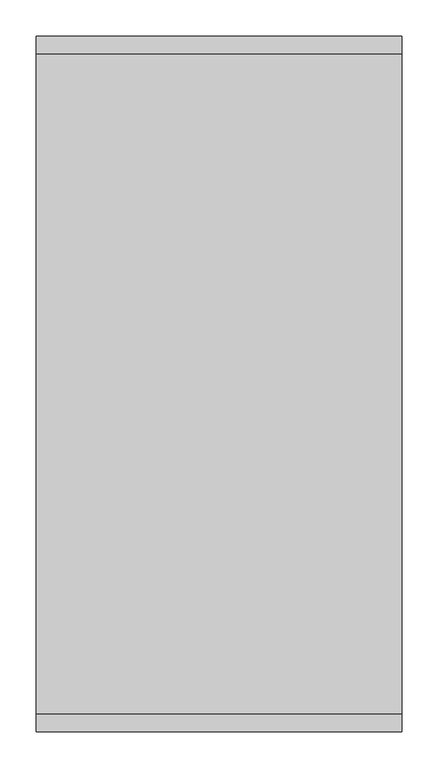
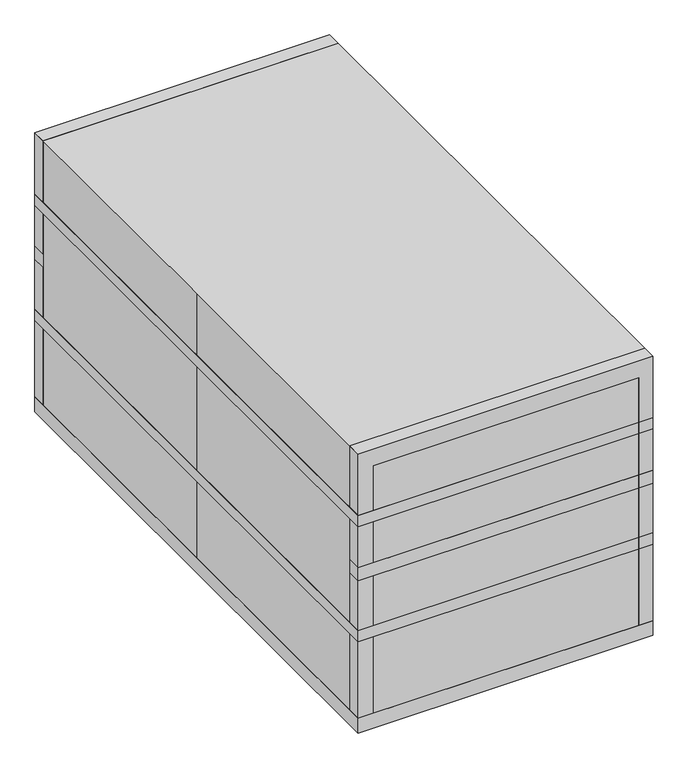
"""IFC4 building model written with IfcOpenShell, lengths in millimetres: proxy geometry, S0290 - Rack, 2SH, 20x20x38 CHMBR : S0290 - Rack, 2SH, 20x20x38 CHMBR."""

import ifcopenshell
import ifcopenshell.guid

model = None  # the IFC model being written
_history = None  # IfcOwnerHistory: only IFC2X3 demands one
_inside = {}  # id of a spatial element -> (the spatial element, [elements in it])
_under = {}  # id of a project, library or spatial element -> (it, [spatial elements below it])
_declared = {}  # id of a project -> (the project, [libraries it declares])
_typed = {}  # id of a type object -> (the type object, [elements of that type])
_made_of = {}  # id of a material, layer set ... -> (it, [elements and type objects made of it])


def new_model(schema):
    """Start an empty IFC model of exactly this schema.

    Asked for "IFC4X3", IfcOpenShell would pick the latest addendum, in which some entities
    have other attributes; the version numbers below select the first issue.
    IFC2X3 requires an IfcOwnerHistory on every rooted entity: one is made here for all.
    """
    global model, _history
    if schema == "IFC4X3":
        model = ifcopenshell.file(schema_version=(4, 3, 0, 0))
    else:
        model = ifcopenshell.file(schema=schema)
    _inside.clear()
    _under.clear()
    _declared.clear()
    _typed.clear()
    _made_of.clear()
    _history = None
    if model.schema == "IFC2X3":
        org = make("IfcOrganization", Name="unknown")
        user = make(
            "IfcPersonAndOrganization",
            ThePerson=make("IfcPerson", FamilyName="unknown"),
            TheOrganization=org,
        )
        app = make(
            "IfcApplication",
            ApplicationDeveloper=org,
            Version="unknown",
            ApplicationFullName="unknown",
            ApplicationIdentifier="unknown",
        )
        _history = make(
            "IfcOwnerHistory",
            OwningUser=user,
            OwningApplication=app,
            ChangeAction="ADDED",
            CreationDate=0,
        )
    return model


def make(cls, **values):
    """One entity of the class cls with the attributes given. An attribute that is None is left unset."""
    return model.create_entity(
        cls, **{name: value for name, value in values.items() if value is not None}
    )


def rooted(cls, **values):
    """An entity with a GlobalId (a new one), such as an element, a storey or a relation."""
    return make(cls, GlobalId=ifcopenshell.guid.new(), OwnerHistory=_history, **values)


def si_unit(unit_type, name, prefix=None):
    """IfcSIUnit, for example si_unit("LENGTHUNIT", "METRE", prefix="MILLI")."""
    return make("IfcSIUnit", UnitType=unit_type, Prefix=prefix, Name=name)


def assignment(units):
    """IfcUnitAssignment: the units of a project."""
    return None if units is None else make("IfcUnitAssignment", Units=units)


def point(xyz):
    """IfcCartesianPoint."""
    return None if xyz is None else make("IfcCartesianPoint", Coordinates=xyz)


def direction(xyz):
    """IfcDirection."""
    return None if xyz is None else make("IfcDirection", DirectionRatios=xyz)


def frame(location, z_axis=None, x_axis=None):
    """IfcAxis2Placement3D, a coordinate frame: its origin and axes. An axis left out is left unset."""
    return make(
        "IfcAxis2Placement3D",
        Location=point(location),
        Axis=direction(z_axis),
        RefDirection=direction(x_axis),
    )


def origin():
    """The frame at (0, 0, 0) with its axes left unset."""
    return frame((0.0, 0.0, 0.0))


def origin_with_axes():
    """The frame at (0, 0, 0) with the z axis (0, 0, 1) and the x axis (1, 0, 0) written out."""
    return frame((0.0, 0.0, 0.0), z_axis=(0.0, 0.0, 1.0), x_axis=(1.0, 0.0, 0.0))


def place(relative_to, where):
    """IfcLocalPlacement: puts the frame where relative to a parent placement (None: the world)."""
    return make(
        "IfcLocalPlacement", PlacementRelTo=relative_to, RelativePlacement=where
    )


def context(
    kind, dimensions, precision=None, world=None, true_north=None, identifier=None
):
    """IfcGeometricRepresentationContext, for example the 3D "Model" context."""
    return make(
        "IfcGeometricRepresentationContext",
        ContextIdentifier=identifier,
        ContextType=kind,
        CoordinateSpaceDimension=dimensions,
        Precision=precision,
        WorldCoordinateSystem=world,
        TrueNorth=true_north,
    )


def project(units=None, contexts=None):
    """IfcProject with its units and contexts."""
    return rooted(
        "IfcProject",
        Name="project",
        RepresentationContexts=contexts,
        UnitsInContext=assignment(units),
    )


def spatial(cls, under=None, at=None, **own):
    """A site, building, storey or space (cls), placed at a placement, below another one or the project."""
    s = rooted(cls, ObjectPlacement=at, **own)
    if under is not None:
        _under.setdefault(under.id(), (under, []))[1].append(s)
    return s


def polyline(points):
    """IfcPolyline through the points."""
    return make("IfcPolyline", Points=[point(p) for p in points])


def outline(outer, holes=None, kind="AREA"):
    """IfcArbitraryClosedProfileDef: a profile drawn as a closed curve; with holes, ...WithVoids."""
    if holes is None:
        return make("IfcArbitraryClosedProfileDef", ProfileType=kind, OuterCurve=outer)
    return make(
        "IfcArbitraryProfileDefWithVoids",
        ProfileType=kind,
        OuterCurve=outer,
        InnerCurves=holes,
    )


def extrude(swept, where, along, depth):
    """IfcExtrudedAreaSolid: the profile swept, set in the frame where, extruded along a direction by depth."""
    return make(
        "IfcExtrudedAreaSolid",
        SweptArea=swept,
        Position=where,
        ExtrudedDirection=direction(along),
        Depth=depth,
    )


def shape(context_of_items, identifier, shape_type, items):
    """IfcShapeRepresentation: the items that make up one representation, for example the "Body"."""
    return make(
        "IfcShapeRepresentation",
        ContextOfItems=context_of_items,
        RepresentationIdentifier=identifier,
        RepresentationType=shape_type,
        Items=items,
    )


def source(mapping_origin, context_of_items, identifier, shape_type, items):
    """IfcRepresentationMap: a shape defined once, which mapped items show again and again."""
    return make(
        "IfcRepresentationMap",
        MappingOrigin=mapping_origin,
        MappedRepresentation=shape(context_of_items, identifier, shape_type, items),
    )


def transform(
    local_origin,
    x_axis=None,
    y_axis=None,
    z_axis=None,
    scale=None,
    scale2=None,
    scale3=None,
    uniform=True,
):
    """IfcCartesianTransformationOperator3D, or its non-uniform kind. x_axis, y_axis, z_axis: its Axis1, 2, 3."""
    if uniform:
        return make(
            "IfcCartesianTransformationOperator3D",
            Axis1=direction(x_axis),
            Axis2=direction(y_axis),
            LocalOrigin=point(local_origin),
            Scale=scale,
            Axis3=direction(z_axis),
        )
    return make(
        "IfcCartesianTransformationOperator3DnonUniform",
        Axis1=direction(x_axis),
        Axis2=direction(y_axis),
        LocalOrigin=point(local_origin),
        Scale=scale,
        Axis3=direction(z_axis),
        Scale2=scale2,
        Scale3=scale3,
    )


def mapped(mapping_source, mapping_target):
    """IfcMappedItem: shows the shape of a source again, moved by a transform."""
    return make(
        "IfcMappedItem", MappingSource=mapping_source, MappingTarget=mapping_target
    )


def made_of(thing, what):
    """Note that an element or type object is made of a material, layer set ...; save() writes the relation."""
    if what is not None:
        _made_of.setdefault(what.id(), (what, []))[1].append(thing)
    return thing


def element(
    cls,
    number,
    at=None,
    inside=None,
    cuts=None,
    type_object=None,
    material=None,
    context=None,
    identifier="Body",
    shape_type=None,
    held_by="IfcProductDefinitionShape",
    body=None,
    shapes=None,
    **own,
):
    """One element of the class cls, such as IfcWall. Its Tag is "e" and its number.

    at: its placement. inside: the storey or other place that contains it. cuts: it is an
    opening in that element (IfcRelVoidsElement). A single representation is given by context,
    identifier, shape_type and body (its items); several are given by shapes. held_by: the class
    of the entity that holds the representations. save() writes the other relations.
    """
    e = rooted(cls, Tag="e%d" % number, ObjectPlacement=at, **own)
    if body is not None:
        shapes = [shape(context, identifier, shape_type, body)]
    if shapes is not None:
        e.Representation = make(held_by, Representations=shapes)
    if inside is not None:
        _inside.setdefault(inside.id(), (inside, []))[1].append(e)
    if cuts is not None:
        rooted(
            "IfcRelVoidsElement", RelatingBuildingElement=cuts, RelatedOpeningElement=e
        )
    if type_object is not None:
        _typed.setdefault(type_object.id(), (type_object, []))[1].append(e)
    return made_of(e, material)


def aggregate(whole, parts):
    """IfcRelAggregates: a whole, such as a stair, and the parts it consists of."""
    return rooted("IfcRelAggregates", RelatingObject=whole, RelatedObjects=parts)


def save(model, path):
    """Write the relations noted so far, then the file.

    IfcRelAggregates (storeys below a building ...), IfcRelContainedInSpatialStructure (elements
    in a storey), IfcRelDefinesByType, IfcRelAssociatesMaterial and IfcRelDeclares: one each for
    every whole, place, type object, material and project.
    """
    for whole, parts in _under.values():
        aggregate(whole, parts)
    for where, things in _inside.values():
        rooted(
            "IfcRelContainedInSpatialStructure",
            RelatedElements=things,
            RelatingStructure=where,
        )
    for kind, things in _typed.values():
        rooted("IfcRelDefinesByType", RelatedObjects=things, RelatingType=kind)
    for what, things in _made_of.values():
        rooted("IfcRelAssociatesMaterial", RelatedObjects=things, RelatingMaterial=what)
    for by, libraries in _declared.values():
        rooted("IfcRelDeclares", RelatingContext=by, RelatedDefinitions=libraries)
    model.write(path)


def specialty_equipment_4a336ec8(model_context):
    return source(origin(), model_context, "Body", "SweptSolid", [
        extrude(outline(polyline([(254.0, 482.6), (254.0, 458.0324286), (-254.0, 458.0324286), (-254.0, 482.6), (254.0, 482.6)])), frame((0.0, 0.0, 277.4471471), z_axis=(0.0, 0.0, 1.0), x_axis=(1.0, 0.0, 0.0)), (0.0, 0.0, 1.0), 23.2707904),
        extrude(outline(polyline([(254.0, -458.0324286), (254.0, -482.6), (-254.0, -482.6), (-254.0, -458.0324286), (254.0, -458.0324286)])), frame((0.0, 0.0, 277.4471471), z_axis=(0.0, 0.0, 1.0), x_axis=(1.0, 0.0, 0.0)), (0.0, 0.0, 1.0), 23.2707904),
        extrude(outline(polyline([(254.0, -482.6), (-254.0, -482.6), (-254.0, 482.6), (254.0, 482.6), (254.0, -482.6)])), frame((0.0, 0.0, 375.8767366), z_axis=(0.0, 0.0, 1.0), x_axis=(1.0, 0.0, 0.0)), (0.0, 0.0, 1.0), 20.120207),
        extrude(outline(polyline([(254.0, -482.6), (-254.0, -482.6), (-254.0, 482.6), (254.0, 482.6), (254.0, -482.6)])), frame((0.0, 0.0, 166.3267366), z_axis=(0.0, 0.0, 1.0), x_axis=(1.0, 0.0, 0.0)), (0.0, 0.0, 1.0), 20.120207),
        extrude(outline(polyline([(229.2176472, 19.308138), (229.2176472, -18.1308753), (-227.8503058, -18.1308753), (-227.8503058, 19.308138), (229.2176472, 19.308138)])), origin_with_axes(), (0.0, 0.0, 1.0), 26.7236401),
        extrude(outline(polyline([(254.0, 482.6), (254.0, -482.6), (-254.0, -482.6), (-254.0, 482.6), (254.0, 482.6)]), holes=[polyline([(229.2176472, 458.0324286), (-227.8503058, 458.0324286), (-227.8503058, -458.0324286), (229.2176472, -458.0324286), (229.2176472, 458.0324286)])]), origin_with_axes(), (0.0, 0.0, 1.0), 26.7236401),
        extrude(outline(polyline([(508.0, 254.0), (508.0, -254.0), (0.0, -254.0), (0.0, 254.0), (508.0, 254.0)]), holes=[polyline([(477.4604177, 229.2176472), (26.7236401, 229.2176472), (26.7236401, -227.8503058), (477.4604177, -227.8503058), (477.4604177, 229.2176472)])]), frame((0.0, 458.0324286, 0.0), z_axis=(0.0, 1.0, 0.0), x_axis=(0.0, 0.0, 1.0)), (0.0, 0.0, 1.0), 24.5675714),
        extrude(outline(polyline([(508.0, 254.0), (508.0, -254.0), (0.0, -254.0), (0.0, 254.0), (508.0, 254.0)]), holes=[polyline([(477.4604177, 229.2176472), (26.7236401, 229.2176472), (26.7236401, -227.8503058), (477.4604177, -227.8503058), (477.4604177, 229.2176472)])]), frame((0.0, -482.6, 0.0), z_axis=(0.0, 1.0, 0.0), x_axis=(0.0, 0.0, 1.0)), (0.0, 0.0, 1.0), 24.5675714),
        extrude(outline(polyline([(-254.0, 482.6), (254.0, 482.6), (254.0, -482.6), (-254.0, -482.6), (-254.0, 0.0), (-254.0, 482.6)])), origin_with_axes(), (0.0, 0.0, 1.0), 508.0),
    ])


if __name__ == "__main__":
    model = new_model("IFC4")
    model_context = context("Model", 3, world=origin())
    ifc_project = project(units=[si_unit("LENGTHUNIT", "METRE", prefix="MILLI")], contexts=[model_context])
    site = spatial("IfcSite", under=ifc_project)
    building = spatial("IfcBuilding", under=site)
    placement = place(None, origin())
    specialty_equipment_shape = specialty_equipment_4a336ec8(model_context)
    element("IfcBuildingElementProxy", 1, Name="S0290 - Rack, 2SH, 20x20x38 CHMBR : S0290 - Rack, 2SH, 20x20x38 CHMBR", ObjectType="S0290 - Rack, 2SH, 20x20x38 CHMBR : S0290 - Rack, 2SH, 20x20x38 CHMBR", at=placement, inside=building, context=model_context, shape_type="MappedRepresentation", body=[
        mapped(specialty_equipment_shape, transform((0.0, 0.0, 0.0), x_axis=(1.0, 0.0, 0.0), y_axis=(0.0, 1.0, 0.0), z_axis=(0.0, 0.0, 1.0))),
    ])
    save(model, "model.ifc")

# Revit data of these elements
# Type "S0290 - Rack, 2SH, 20x20x38 CHMBR : S0290 - Rack, 2SH, 20x20x38 CHMBR"
#   JSN = "S0290"
#   Nomenclature = "Rack, 2SH, 20x20x38 CHMBR"
#   Utility_6 = "-"
#   Utility_5 = "-"
#   Utility_4 = "-"
#   Utility_3 = "-"
#   Utility_2 = "-"
#   Utility_1 = "-"
#   Unit_Issue = "EA"
#   Price_Date = "0"
#   Nomenclature = "Rack, 2SH, 20x20x38 CHMBR"
#   NSN = "6530"
#   Location [instance default] = ""
#   JSN_Name = "S0290"
#   Hertz_swit = "0"
#   Hertz_dep = "0"
#   Hertz = "0"
#   Desc = "Rack with two extendable shelves for use with sterilizers having a 20X20X38 chamber. For use in providing loading efficiency for a wide variety of mixed or single item loads."
#   CAT_VA = "-"
#   CAT_Navy = "A"
#   CAT_IHS = "A"
#   CAT_Army = "A"
#   CAT_AF = "-"
#   BTUPerHour = "0"
#   Width_IN = 0
#   Weight_AV = 18
#   Watts2 = 0
#   Watts1 = 0
#   Volts2 = 0
#   Volts1 = 0
#   Phase2 = 0
#   Phase1 = 0
#   Height_IN = 0
#   Depth_IN = 0
#   Amps2 = 0
#   Amps1 = 0
# Element 1 (IfcBuildingElementProxy, "S0290 - Rack, 2SH, 20x20x38 CHMBR : S0290 - Rack, 2SH, 20x20x38 CHMBR")
#   Materials on its faces: "EquipSpace"
# Materials
#   "EquipSpace": class "Unassigned", colour RGB 221 217 195, transparency 0.5
